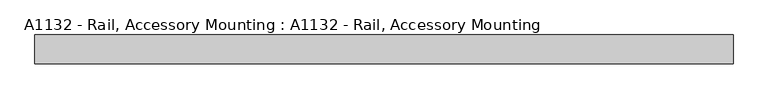
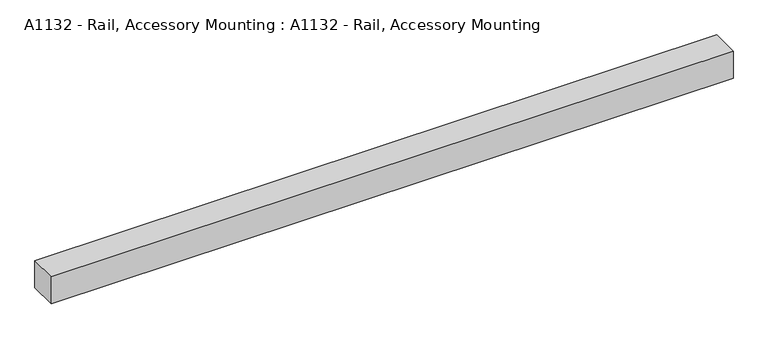
"""IFC4 building model written with IfcOpenShell, lengths in millimetres: proxy geometry, A1132 - Rail, Accessory Mounting : A1132 - Rail, Accessory Mounting."""

import ifcopenshell
import ifcopenshell.guid

model = None  # the IFC model being written
_history = None  # IfcOwnerHistory: only IFC2X3 demands one
_inside = {}  # id of a spatial element -> (the spatial element, [elements in it])
_under = {}  # id of a project, library or spatial element -> (it, [spatial elements below it])
_declared = {}  # id of a project -> (the project, [libraries it declares])
_typed = {}  # id of a type object -> (the type object, [elements of that type])
_made_of = {}  # id of a material, layer set ... -> (it, [elements and type objects made of it])


def new_model(schema):
    """Start an empty IFC model of exactly this schema.

    Asked for "IFC4X3", IfcOpenShell would pick the latest addendum, in which some entities
    have other attributes; the version numbers below select the first issue.
    IFC2X3 requires an IfcOwnerHistory on every rooted entity: one is made here for all.
    """
    global model, _history
    if schema == "IFC4X3":
        model = ifcopenshell.file(schema_version=(4, 3, 0, 0))
    else:
        model = ifcopenshell.file(schema=schema)
    _inside.clear()
    _under.clear()
    _declared.clear()
    _typed.clear()
    _made_of.clear()
    _history = None
    if model.schema == "IFC2X3":
        org = make("IfcOrganization", Name="unknown")
        user = make(
            "IfcPersonAndOrganization",
            ThePerson=make("IfcPerson", FamilyName="unknown"),
            TheOrganization=org,
        )
        app = make(
            "IfcApplication",
            ApplicationDeveloper=org,
            Version="unknown",
            ApplicationFullName="unknown",
            ApplicationIdentifier="unknown",
        )
        _history = make(
            "IfcOwnerHistory",
            OwningUser=user,
            OwningApplication=app,
            ChangeAction="ADDED",
            CreationDate=0,
        )
    return model


def make(cls, **values):
    """One entity of the class cls with the attributes given. An attribute that is None is left unset."""
    return model.create_entity(
        cls, **{name: value for name, value in values.items() if value is not None}
    )


def rooted(cls, **values):
    """An entity with a GlobalId (a new one), such as an element, a storey or a relation."""
    return make(cls, GlobalId=ifcopenshell.guid.new(), OwnerHistory=_history, **values)


def si_unit(unit_type, name, prefix=None):
    """IfcSIUnit, for example si_unit("LENGTHUNIT", "METRE", prefix="MILLI")."""
    return make("IfcSIUnit", UnitType=unit_type, Prefix=prefix, Name=name)


def assignment(units):
    """IfcUnitAssignment: the units of a project."""
    return None if units is None else make("IfcUnitAssignment", Units=units)


def point(xyz):
    """IfcCartesianPoint."""
    return None if xyz is None else make("IfcCartesianPoint", Coordinates=xyz)


def direction(xyz):
    """IfcDirection."""
    return None if xyz is None else make("IfcDirection", DirectionRatios=xyz)


def frame(location, z_axis=None, x_axis=None):
    """IfcAxis2Placement3D, a coordinate frame: its origin and axes. An axis left out is left unset."""
    return make(
        "IfcAxis2Placement3D",
        Location=point(location),
        Axis=direction(z_axis),
        RefDirection=direction(x_axis),
    )


def origin():
    """The frame at (0, 0, 0) with its axes left unset."""
    return frame((0.0, 0.0, 0.0))


def origin_with_axes():
    """The frame at (0, 0, 0) with the z axis (0, 0, 1) and the x axis (1, 0, 0) written out."""
    return frame((0.0, 0.0, 0.0), z_axis=(0.0, 0.0, 1.0), x_axis=(1.0, 0.0, 0.0))


def place(relative_to, where):
    """IfcLocalPlacement: puts the frame where relative to a parent placement (None: the world)."""
    return make(
        "IfcLocalPlacement", PlacementRelTo=relative_to, RelativePlacement=where
    )


def context(
    kind, dimensions, precision=None, world=None, true_north=None, identifier=None
):
    """IfcGeometricRepresentationContext, for example the 3D "Model" context."""
    return make(
        "IfcGeometricRepresentationContext",
        ContextIdentifier=identifier,
        ContextType=kind,
        CoordinateSpaceDimension=dimensions,
        Precision=precision,
        WorldCoordinateSystem=world,
        TrueNorth=true_north,
    )


def project(units=None, contexts=None):
    """IfcProject with its units and contexts."""
    return rooted(
        "IfcProject",
        Name="project",
        RepresentationContexts=contexts,
        UnitsInContext=assignment(units),
    )


def spatial(cls, under=None, at=None, **own):
    """A site, building, storey or space (cls), placed at a placement, below another one or the project."""
    s = rooted(cls, ObjectPlacement=at, **own)
    if under is not None:
        _under.setdefault(under.id(), (under, []))[1].append(s)
    return s


def polyline(points):
    """IfcPolyline through the points."""
    return make("IfcPolyline", Points=[point(p) for p in points])


def outline(outer, holes=None, kind="AREA"):
    """IfcArbitraryClosedProfileDef: a profile drawn as a closed curve; with holes, ...WithVoids."""
    if holes is None:
        return make("IfcArbitraryClosedProfileDef", ProfileType=kind, OuterCurve=outer)
    return make(
        "IfcArbitraryProfileDefWithVoids",
        ProfileType=kind,
        OuterCurve=outer,
        InnerCurves=holes,
    )


def extrude(swept, where, along, depth):
    """IfcExtrudedAreaSolid: the profile swept, set in the frame where, extruded along a direction by depth."""
    return make(
        "IfcExtrudedAreaSolid",
        SweptArea=swept,
        Position=where,
        ExtrudedDirection=direction(along),
        Depth=depth,
    )


def shape(context_of_items, identifier, shape_type, items):
    """IfcShapeRepresentation: the items that make up one representation, for example the "Body"."""
    return make(
        "IfcShapeRepresentation",
        ContextOfItems=context_of_items,
        RepresentationIdentifier=identifier,
        RepresentationType=shape_type,
        Items=items,
    )


def source(mapping_origin, context_of_items, identifier, shape_type, items):
    """IfcRepresentationMap: a shape defined once, which mapped items show again and again."""
    return make(
        "IfcRepresentationMap",
        MappingOrigin=mapping_origin,
        MappedRepresentation=shape(context_of_items, identifier, shape_type, items),
    )


def transform(
    local_origin,
    x_axis=None,
    y_axis=None,
    z_axis=None,
    scale=None,
    scale2=None,
    scale3=None,
    uniform=True,
):
    """IfcCartesianTransformationOperator3D, or its non-uniform kind. x_axis, y_axis, z_axis: its Axis1, 2, 3."""
    if uniform:
        return make(
            "IfcCartesianTransformationOperator3D",
            Axis1=direction(x_axis),
            Axis2=direction(y_axis),
            LocalOrigin=point(local_origin),
            Scale=scale,
            Axis3=direction(z_axis),
        )
    return make(
        "IfcCartesianTransformationOperator3DnonUniform",
        Axis1=direction(x_axis),
        Axis2=direction(y_axis),
        LocalOrigin=point(local_origin),
        Scale=scale,
        Axis3=direction(z_axis),
        Scale2=scale2,
        Scale3=scale3,
    )


def mapped(mapping_source, mapping_target):
    """IfcMappedItem: shows the shape of a source again, moved by a transform."""
    return make(
        "IfcMappedItem", MappingSource=mapping_source, MappingTarget=mapping_target
    )


def made_of(thing, what):
    """Note that an element or type object is made of a material, layer set ...; save() writes the relation."""
    if what is not None:
        _made_of.setdefault(what.id(), (what, []))[1].append(thing)
    return thing


def element(
    cls,
    number,
    at=None,
    inside=None,
    cuts=None,
    type_object=None,
    material=None,
    context=None,
    identifier="Body",
    shape_type=None,
    held_by="IfcProductDefinitionShape",
    body=None,
    shapes=None,
    **own,
):
    """One element of the class cls, such as IfcWall. Its Tag is "e" and its number.

    at: its placement. inside: the storey or other place that contains it. cuts: it is an
    opening in that element (IfcRelVoidsElement). A single representation is given by context,
    identifier, shape_type and body (its items); several are given by shapes. held_by: the class
    of the entity that holds the representations. save() writes the other relations.
    """
    e = rooted(cls, Tag="e%d" % number, ObjectPlacement=at, **own)
    if body is not None:
        shapes = [shape(context, identifier, shape_type, body)]
    if shapes is not None:
        e.Representation = make(held_by, Representations=shapes)
    if inside is not None:
        _inside.setdefault(inside.id(), (inside, []))[1].append(e)
    if cuts is not None:
        rooted(
            "IfcRelVoidsElement", RelatingBuildingElement=cuts, RelatedOpeningElement=e
        )
    if type_object is not None:
        _typed.setdefault(type_object.id(), (type_object, []))[1].append(e)
    return made_of(e, material)


def aggregate(whole, parts):
    """IfcRelAggregates: a whole, such as a stair, and the parts it consists of."""
    return rooted("IfcRelAggregates", RelatingObject=whole, RelatedObjects=parts)


def save(model, path):
    """Write the relations noted so far, then the file.

    IfcRelAggregates (storeys below a building ...), IfcRelContainedInSpatialStructure (elements
    in a storey), IfcRelDefinesByType, IfcRelAssociatesMaterial and IfcRelDeclares: one each for
    every whole, place, type object, material and project.
    """
    for whole, parts in _under.values():
        aggregate(whole, parts)
    for where, things in _inside.values():
        rooted(
            "IfcRelContainedInSpatialStructure",
            RelatedElements=things,
            RelatingStructure=where,
        )
    for kind, things in _typed.values():
        rooted("IfcRelDefinesByType", RelatedObjects=things, RelatingType=kind)
    for what, things in _made_of.values():
        rooted("IfcRelAssociatesMaterial", RelatedObjects=things, RelatingMaterial=what)
    for by, libraries in _declared.values():
        rooted("IfcRelDeclares", RelatingContext=by, RelatedDefinitions=libraries)
    model.write(path)


def a1132_rail_accessory_mounting_a1132_rail_accessory_mounting_a2e13202(model_context):
    return source(origin(), model_context, "Body", "SweptSolid", [
        extrude(outline(polyline([(609.6, -50.8), (-609.6, -50.8), (-609.6, 0.0), (609.6, 0.0), (609.6, -50.8)])), origin_with_axes(), (0.0, 0.0, 1.0), 50.8),
        extrude(outline(polyline([(-12.7, 25.4), (-12.7, 0.0), (-38.1, 0.0), (-38.1, 25.4), (-50.8, 25.4), (-50.8, 50.8), (0.0, 50.8), (0.0, 25.4), (-12.7, 25.4)])), frame((-609.6, 0.0, 0.0), z_axis=(1.0, 0.0, 0.0), x_axis=(0.0, 1.0, 0.0)), (0.0, 0.0, 1.0), 1219.2),
    ])


if __name__ == "__main__":
    model = new_model("IFC4")
    model_context = context("Model", 3, world=origin())
    ifc_project = project(units=[si_unit("LENGTHUNIT", "METRE", prefix="MILLI")], contexts=[model_context])
    site = spatial("IfcSite", under=ifc_project)
    building = spatial("IfcBuilding", under=site)
    placement = place(None, origin())
    a1132_rail_accessory_mounting_a1132_rail_accessory_mounting_shape = a1132_rail_accessory_mounting_a1132_rail_accessory_mounting_a2e13202(model_context)
    element("IfcBuildingElementProxy", 1, Name="A1132 - Rail, Accessory Mounting : A1132 - Rail, Accessory Mounting", ObjectType="A1132 - Rail, Accessory Mounting : A1132 - Rail, Accessory Mounting", at=placement, inside=building, context=model_context, shape_type="MappedRepresentation", body=[
        mapped(a1132_rail_accessory_mounting_a1132_rail_accessory_mounting_shape, transform((0.0, 0.0, 0.0), x_axis=(1.0, 0.0, 0.0), y_axis=(0.0, 1.0, 0.0), z_axis=(0.0, 0.0, 1.0))),
    ])
    save(model, "model.ifc")

# Revit data of these elements
# Project information
#   Sheets - Total = "6"
#   Project Issue Date = "Issue Date"
#   Project Status = "Project Status"
#   Client Name = "Owner"
#   Project Address = "Enter address here"
#   Project Name = "Project Name"
#   Project Number = "Project Number"
#   Publication Date = "30-Jan-15"
# Type "A1132 - Rail, Accessory Mounting : A1132 - Rail, Accessory Mounting"
#   Watts2 = "0"
#   Watts1 = "0"
#   Unit_Issue = "LF"
#   UTIL_6_Misc = "-"
#   UTIL_5_NonMedGas = "-"
#   UTIL_4_MiscGas = "-"
#   UTIL_3_MedGas = "-"
#   UTIL_2_Elec = "-"
#   UTIL_1_WaterDrain = "-"
#   Nomenclature = "Rail, Accessory Mounting, 48\""
#   NSN = "6530"
#   Location [instance default] = ""
#   JSN = "A1132"
#   Fund_Source_VA = "-"
#   Fund_Source_Navy = "C"
#   Fund_Source_Army = "-"
#   Fund_Source_AF = "-"
#   ELEC_Volts2 = "0"
#   ELEC_Volts1 = "0"
#   ELEC_Phase2 = "0"
#   ELEC_Phase1 = "0"
#   ELEC_HertzSwitch = "0"
#   ELEC_HertzDependent = "0"
#   ELEC_Hertz = "0"
#   ELEC_Amps2 = "0"
#   ELEC_Amps1 = "0"
#   DetailDescription = "Horizontal mounting rail will consist of lock mounting devices capable of; supporting up to 75 pounds each, being repositioned, and mounting and dismounting of equipment without the use of tools. The rail must be capable of supporting medical equipment and accessories normally found in exam or patient rooms. The rail system must be capable of mounting and dismounting equipment without leaving or creating new holes in the finished surface of the wall."
#   CAT_VA = "A"
#   CAT_Navy = "A"
#   CAT_IHS = "-"
#   CAT_Army = "A"
#   CAT_AF = "A"
#   BTUperhour = "0"
#   Weight_IP = 5
#   Default Elevation = 4' - 0"
#   DIM_Width_IP = 4' - 0"
#   DIM_Height_IP = 0' - 2"
#   DIM_Depth_IP = 0' - 2"
#   CustomLength [instance default] = 4' - 0"
#   Assembly Code = ""
# Element 1 (IfcBuildingElementProxy, "A1132 - Rail, Accessory Mounting : A1132 - Rail, Accessory Mounting")
#   Location = "LDAT1"
#   Materials on its faces: "EquipSpace"
# Materials
#   "EquipSpace": class "Unassigned", colour RGB 221 217 195, transparency 0.5
